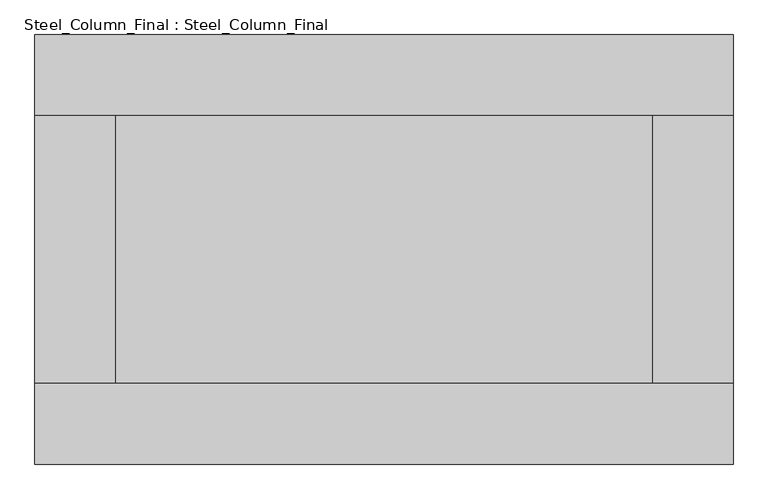
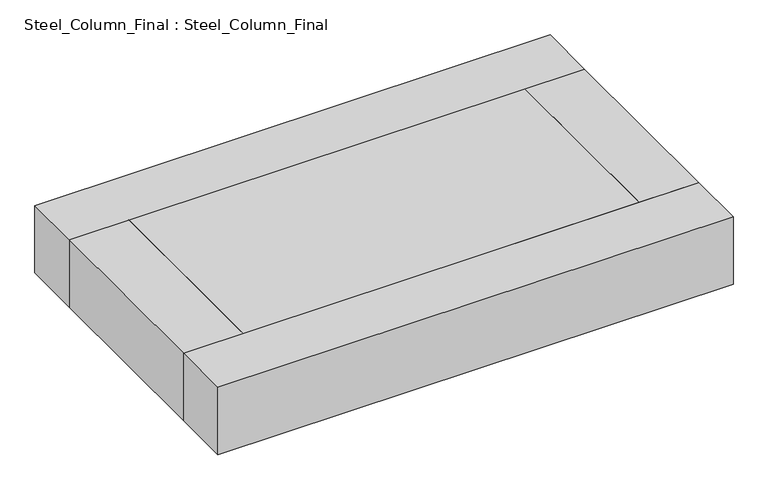
"""IFC4 building model written with IfcOpenShell, lengths in millimetres: proxy geometry, Steel_Column_Final : Steel_Column_Final."""

from ifc_helpers import new_model, si_unit, frame, origin, place, context, project, spatial, polyline, outline, extrude, source, transform, mapped, element, save


def steel_column_final_steel_column_final_81049bd6(model_context):
    return source(origin(), model_context, "Body", "SweptSolid", [
        extrude(outline(polyline([(6500.0, 2500.0), (-6500.0, 2500.0), (-6500.0, 4000.0), (6500.0, 4000.0), (6500.0, 2500.0)])), frame((0.0, 0.0, 130700.0), z_axis=(0.0, 0.0, 1.0), x_axis=(1.0, 0.0, 0.0)), (0.0, 0.0, 1.0), 1800.0),
        extrude(outline(polyline([(-6500.0, -2500.0), (6500.0, -2500.0), (6500.0, -4000.0), (-6500.0, -4000.0), (-6500.0, -2500.0)])), frame((0.0, 0.0, 130700.0), z_axis=(0.0, 0.0, 1.0), x_axis=(1.0, 0.0, 0.0)), (0.0, 0.0, 1.0), 1800.0),
        extrude(outline(polyline([(5000.0, -2500.0), (5000.0, 2500.0), (6500.0, 2500.0), (6500.0, -2500.0), (5000.0, -2500.0)])), frame((0.0, 0.0, 130700.0), z_axis=(0.0, 0.0, 1.0), x_axis=(1.0, 0.0, 0.0)), (0.0, 0.0, 1.0), 1800.0),
        extrude(outline(polyline([(-5000.0, 2500.0), (-5000.0, -2500.0), (-6500.0, -2500.0), (-6500.0, 2500.0), (-5000.0, 2500.0)])), frame((0.0, 0.0, 130700.0), z_axis=(0.0, 0.0, 1.0), x_axis=(1.0, 0.0, 0.0)), (0.0, 0.0, 1.0), 1800.0),
        extrude(outline(polyline([(-5000.0, -2500.0), (-5000.0, 2500.0), (5000.0, 2500.0), (5000.0, -2500.0), (-5000.0, -2500.0)])), frame((0.0, 0.0, 130700.0), z_axis=(0.0, 0.0, 1.0), x_axis=(1.0, 0.0, 0.0)), (0.0, 0.0, 1.0), 1800.0),
    ])


if __name__ == "__main__":
    model = new_model("IFC4")
    model_context = context("Model", 3, world=origin())
    ifc_project = project(units=[si_unit("LENGTHUNIT", "METRE", prefix="MILLI")], contexts=[model_context])
    site = spatial("IfcSite", under=ifc_project)
    building = spatial("IfcBuilding", under=site)
    placement = place(None, origin())
    steel_column_final_steel_column_final_shape = steel_column_final_steel_column_final_81049bd6(model_context)
    element("IfcBuildingElementProxy", 1, Name="Steel_Column_Final : Steel_Column_Final", ObjectType="Steel_Column_Final : Steel_Column_Final", at=placement, inside=building, context=model_context, shape_type="MappedRepresentation", body=[
        mapped(steel_column_final_steel_column_final_shape, transform((0.0, 0.0, 0.0), x_axis=(1.0, 0.0, 0.0), y_axis=(0.0, 1.0, 0.0), z_axis=(0.0, 0.0, 1.0))),
    ])
    save(model, "model.ifc")

# Revit data of these elements
# Type "Steel_Column_Final : Steel_Column_Final"
#   Top Width [instance default] = 5000 mm
#   Top Length = 10000 mm
#   Length = 21000 mm
#   Height [instance default] = 50000 mm
#   Bottom Width [instance default] = 5000 mm
#   Default Elevation = 0
# Element 1 (IfcBuildingElementProxy, "Steel_Column_Final : Steel_Column_Final")
#   Height = 130700 mm
